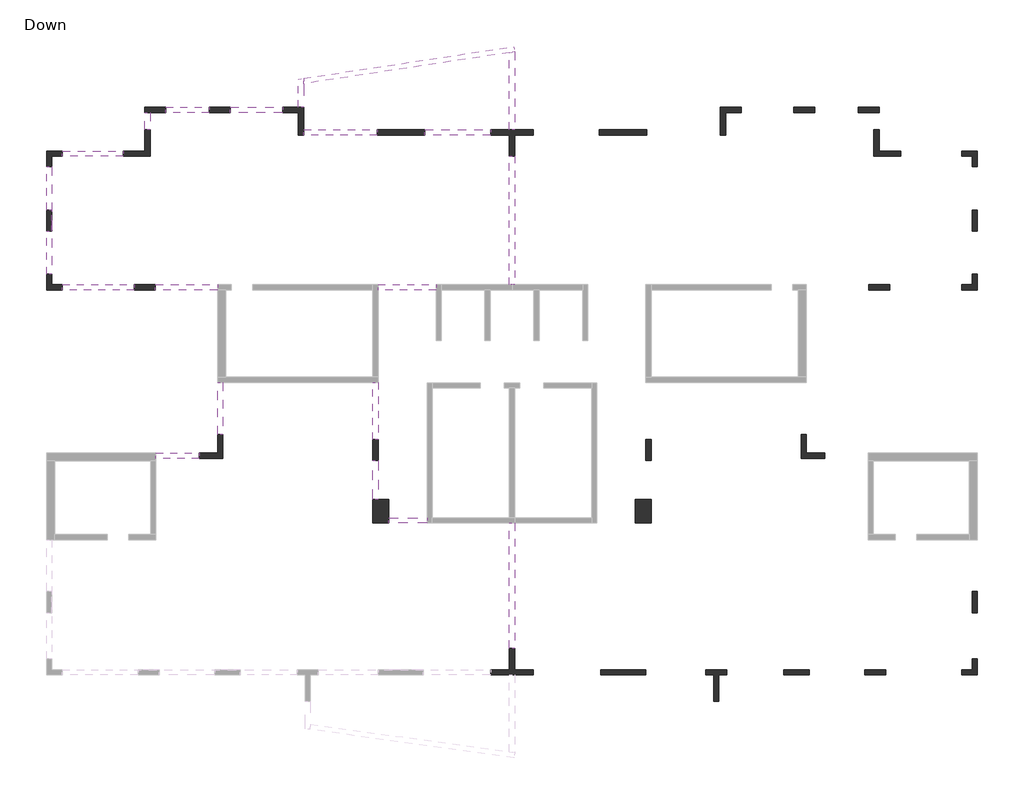
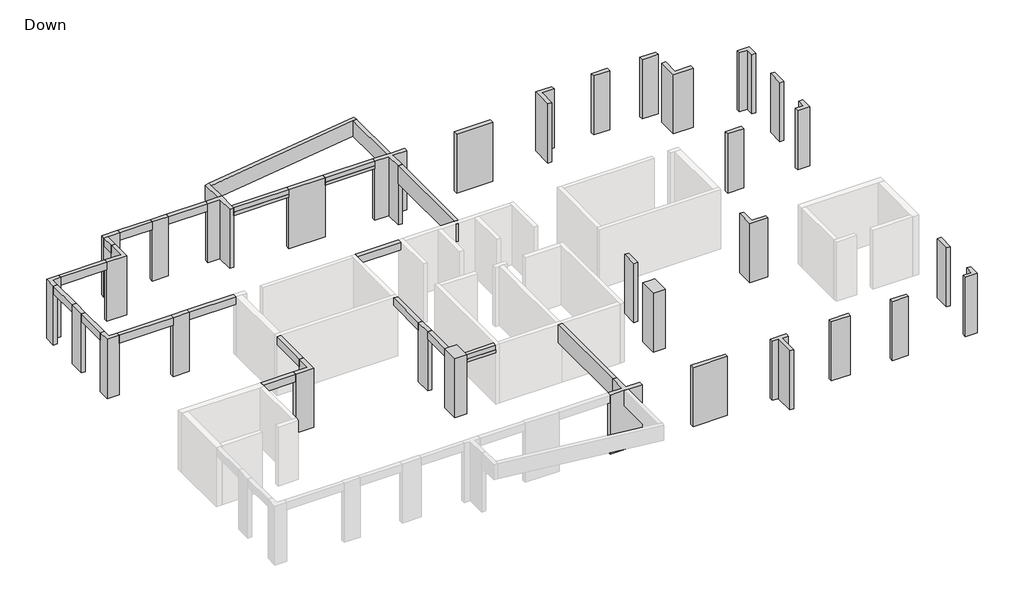
# One storey, part 2 of 2: 32 columns, 21 beams.
"""IFC4 building model written with IfcOpenShell, lengths in millimetres."""

from ifc_helpers import new_model, si_unit, frame, origin, origin_with_axes, place, context, project, spatial, polyline, outline, extrude, faceted_brep, element, save

model = new_model("IFC4")

# Units and contexts
model_context = context("Model", 3, world=origin())
ifc_project = project(units=[si_unit("LENGTHUNIT", "METRE", prefix="MILLI")], contexts=[model_context])

# Site, building, storey
site = spatial("IfcSite", under=ifc_project)
building = spatial("IfcBuilding", under=site)
storey = spatial("IfcBuildingStorey", under=building, Name="Down", Elevation=0.0)

# Beams
placement = place(None, origin())
element("IfcBeam", 1, ObjectType="Concrete Rectengular Beam : 20/40", at=placement, inside=storey, context=model_context, shape_type="Brep", body=[
    faceted_brep([(-16045.271188, -5036.9600972, 3120.0), (-16045.271188, -4836.9600972, 3120.0), (-16045.271188, -4836.9600972, 2720.0), (-16045.271188, -5036.9600972, 2720.0), (-16045.271188, -5036.9600972, 2890.0), (-14415.271188, -5036.9600972, 3120.0), (-14415.271188, -4836.9600972, 3120.0), (-14415.271188, -4836.9600972, 2720.0), (-14415.271188, -5036.9600972, 2720.0), (-14415.271188, -5036.9600972, 2890.0)], [[[0, 1, 2, 3, 4]], [[1, 0, 5, 6]], [[2, 1, 6, 7]], [[3, 2, 7, 8]], [[5, 0, 4, 3, 8, 9]], [[6, 5, 9, 8, 7]]]),
])
element("IfcBeam", 2, ObjectType="Concrete Rectengular Beam : 20/40", at=placement, inside=storey, context=model_context, shape_type="Brep", body=[
    faceted_brep([(-13715.271188, -4136.9600972, 3120.0), (-13515.271188, -4136.9600972, 3120.0), (-13515.271188, -2169.1055386, 3120.0), (-13715.271188, -2169.1055386, 3120.0), (-13515.271188, -4136.9600972, 2890.0), (-13515.271188, -4136.9600972, 2720.0), (-13515.271188, -2169.1055386, 2720.0), (-13515.271188, -2169.1055386, 2890.0), (-13715.271188, -4136.9600972, 2720.0), (-13715.271188, -2169.1055386, 2720.0)], [[[0, 1, 2, 3]], [[2, 1, 4, 5, 6, 7]], [[5, 8, 9, 6]], [[8, 0, 3, 9]], [[1, 0, 8, 5, 4]], [[3, 2, 7, 6, 9]]]),
])
element("IfcBeam", 3, ObjectType="Concrete Rectengular Beam : 20/40", at=placement, inside=storey, context=model_context, shape_type="Brep", body=[
    faceted_brep([(-5816.3023024, -7475.6540191, 2720.0), (-5816.3023024, -7475.1655965, 2720.0), (-5816.3023024, -7475.1655965, 2890.0), (-5816.3023024, -7475.6540191, 2890.0), (-5816.5012893, -7275.6540191, 3120.0), (-7266.3023024, -7275.6540191, 3120.0), (-7266.3023024, -7475.1655965, 3120.0), (-5816.5012893, -7475.1655965, 3120.0), (-7266.3023024, -7475.6540191, 2720.0), (-7266.3023024, -7475.6540191, 2890.0), (-7266.3023024, -7275.6540191, 2720.0), (-5816.5012893, -7275.6540191, 2720.0), (-5816.5012893, -7475.1655965, 2720.0), (-7266.3023024, -7275.6540191, 2890.0), (-5816.5012893, -7275.6540191, 2890.0), (-7266.3023024, -7475.1655965, 2890.0), (-5816.5012893, -7475.1655965, 2890.0)], [[[0, 1, 2, 3]], [[4, 5, 6, 7]], [[8, 0, 3, 9]], [[0, 8, 10, 11, 12, 1]], [[10, 13, 5, 4, 14, 11]], [[10, 8, 9, 15, 6, 5, 13]], [[4, 7, 16, 12, 11, 14]], [[1, 12, 16, 2]], [[16, 15, 9, 3, 2]], [[15, 16, 7, 6]]]),
])
element("IfcBeam", 4, ObjectType="Concrete Rectengular Beam : 20/40", at=placement, inside=storey, context=model_context, shape_type="Brep", body=[
    faceted_brep([(-7866.3203921, -6575.6540191, 3120.0), (-7666.3203921, -6575.6540191, 3120.0), (-7666.3203921, -5121.583831, 3120.0), (-7866.3203921, -5121.583831, 3120.0), (-7666.3203921, -6575.6540191, 2890.0), (-7666.3203921, -6575.6540191, 2720.0), (-7666.3203921, -5121.583831, 2720.0), (-7866.3203921, -6575.6540191, 2720.0), (-7866.3203921, -5121.583831, 2720.0), (-7866.3203921, -5121.583831, 2890.0), (-7866.3203921, -6575.6540191, 2890.0)], [[[0, 1, 2, 3]], [[1, 4, 5, 6, 2]], [[5, 7, 8, 6]], [[0, 3, 9, 8, 7, 10]], [[3, 2, 6, 8, 9]], [[1, 0, 10, 7, 5, 4]]]),
])
element("IfcBeam", 5, ObjectType="Concrete Rectengular Beam : 20/40", at=placement, inside=storey, context=model_context, shape_type="Brep", body=[
    faceted_brep([(-7866.3203921, -4321.583831, 3120.0), (-7666.3203921, -4321.583831, 3120.0), (-7666.3203921, -2169.1055386, 3120.0), (-7866.3203921, -2169.1055386, 3120.0), (-7666.3203921, -4321.583831, 2720.0), (-7666.3203921, -2169.1055386, 2720.0), (-7866.3203921, -4321.583831, 2720.0), (-7866.3203921, -2169.1055386, 2720.0), (-7866.3203921, -2169.1055386, 2890.0), (-7866.3203921, -4321.583831, 2890.0)], [[[0, 1, 2, 3]], [[1, 4, 5, 2]], [[4, 6, 7, 5]], [[0, 3, 8, 7, 6, 9]], [[1, 0, 9, 6, 4]], [[3, 2, 5, 7, 8]]]),
])
element("IfcBeam", 6, ObjectType="Concrete Rectengular Beam : 20/40", at=placement, inside=storey, context=model_context, shape_type="Brep", body=[
    faceted_brep([(-5479.9781345, 1313.6006842, 3120.0), (-5479.9781345, 1513.6006842, 3120.0), (-7666.3203921, 1513.6006842, 3120.0), (-7666.3203921, 1313.6006842, 3120.0), (-5479.9781345, 1313.6006842, 2720.0), (-5479.9781345, 1313.6006842, 2890.0), (-7666.3203921, 1313.6006842, 2890.0), (-7666.3203921, 1313.6006842, 2720.0), (-5479.9781345, 1513.6006842, 2720.0), (-7666.3203921, 1513.6006842, 2720.0), (-5479.9781345, 1513.6006842, 2890.0), (-7666.3203921, 1513.6006842, 2890.0)], [[[0, 1, 2, 3]], [[4, 5, 0, 3, 6, 7]], [[8, 4, 7, 9]], [[2, 1, 10, 8, 9, 11]], [[3, 2, 11, 9, 7, 6]], [[1, 0, 5, 4, 8, 10]]]),
])
element("IfcBeam", 7, ObjectType="Concrete Rectengular Beam : 20/40", at=placement, inside=storey, context=model_context, shape_type="Brep", body=[
    faceted_brep([(-16862.5034601, 1314.1252863, 3120.0), (-16862.5034601, 1514.1252863, 3120.0), (-19564.2400737, 1514.1252863, 3120.0), (-19564.2400737, 1314.1252863, 3120.0), (-16862.5034601, 1314.1252863, 2720.0), (-19564.2400737, 1314.1252863, 2720.0), (-16862.5034601, 1514.1252863, 2720.0), (-19564.2400737, 1514.1252863, 2720.0), (-16862.5034601, 1514.1252863, 2890.0)], [[[0, 1, 2, 3]], [[4, 0, 3, 5]], [[6, 4, 5, 7]], [[1, 8, 6, 7, 2]], [[1, 0, 4, 6, 8]], [[3, 2, 7, 5]]]),
])
element("IfcBeam", 8, ObjectType="Concrete Rectengular Beam : 20/40", at=placement, inside=storey, context=model_context, shape_type="Brep", body=[
    faceted_brep([(-16062.5034601, 1514.1252863, 3120.0), (-16062.5034601, 1314.1252863, 3120.0), (-13715.271188, 1314.1252863, 3120.0), (-13715.271188, 1514.1252863, 3120.0), (-16062.5034601, 1314.1252863, 2720.0), (-13715.271188, 1314.1252863, 2720.0), (-16062.5034601, 1514.1252863, 2720.0), (-13715.271188, 1514.1252863, 2720.0), (-13715.271188, 1514.1252863, 2890.0), (-16062.5034601, 1514.1252863, 2890.0)], [[[0, 1, 2, 3]], [[1, 4, 5, 2]], [[4, 6, 7, 5]], [[0, 3, 8, 7, 6, 9]], [[1, 0, 9, 6, 4]], [[3, 2, 5, 7, 8]]]),
])
element("IfcBeam", 9, ObjectType="Concrete Rectengular Beam : 20/40", at=placement, inside=storey, context=model_context, shape_type="Brep", body=[
    faceted_brep([(-19969.2400737, 3539.1252863, 3120.0), (-20164.2400737, 3539.1252863, 3120.0), (-20164.2400737, 1914.1252863, 3120.0), (-19969.2400737, 1914.1252863, 3120.0), (-19964.2400737, 3934.6498883, 2720.0), (-19964.2400737, 3934.6498883, 2890.0), (-19964.2400737, 1914.1252863, 2890.0), (-19964.2400737, 1914.1252863, 2720.0), (-19965.2892778, 3934.6498883, 2720.0), (-20164.2400737, 1914.1252863, 2720.0), (-20164.2400737, 3539.1252863, 2720.0), (-19965.2892778, 3539.1252863, 2720.0), (-19965.2892778, 3934.6498883, 2890.0), (-19965.2892778, 3539.1252863, 2890.0), (-19969.2400737, 3539.1252863, 2890.0), (-19969.2400737, 1914.1252863, 2890.0)], [[[0, 1, 2, 3]], [[4, 5, 6, 7]], [[8, 4, 7, 9, 10, 11]], [[1, 10, 9, 2]], [[4, 8, 12, 5]], [[8, 11, 13, 12]], [[11, 10, 1, 0, 14, 13]], [[5, 12, 13, 14, 15, 6]], [[14, 0, 3, 15]], [[3, 2, 9, 7, 6, 15]]]),
])
element("IfcBeam", 10, ObjectType="Concrete Rectengular Beam : 20/40", at=placement, inside=storey, context=model_context, shape_type="Brep", body=[
    faceted_brep([(-20164.2400737, 5963.5645048, 3120.0), (-20164.2400737, 4339.1252863, 3120.0), (-19969.2400737, 4339.1252863, 3120.0), (-19969.2400737, 5963.5645048, 3120.0), (-19964.2400737, 3934.6498883, 2720.0), (-19964.2400737, 5963.5645048, 2720.0), (-19964.2400737, 5963.5645048, 2890.0), (-19964.2400737, 3934.6498883, 2890.0), (-19965.2892778, 3934.6498883, 2720.0), (-19965.2892778, 4339.1252863, 2720.0), (-20164.2400737, 4339.1252863, 2720.0), (-20164.2400737, 5963.5645048, 2720.0), (-19965.2892778, 3934.6498883, 2890.0), (-19969.2400737, 5963.5645048, 2890.0), (-19965.2892778, 4339.1252863, 2890.0), (-19969.2400737, 4339.1252863, 2890.0)], [[[0, 1, 2, 3]], [[4, 5, 6, 7]], [[5, 4, 8, 9, 10, 11]], [[0, 11, 10, 1]], [[8, 4, 7, 12]], [[5, 11, 0, 3, 13, 6]], [[10, 9, 14, 15, 2, 1]], [[9, 8, 12, 14]], [[13, 15, 14, 12, 7, 6]], [[15, 13, 3, 2]]]),
])
element("IfcBeam", 11, ObjectType="Concrete Rectengular Beam : 20/40", at=placement, inside=storey, context=model_context, shape_type="Brep", body=[
    faceted_brep([(-19564.2400737, 6563.5645048, 3120.0), (-19564.2400737, 6363.5645048, 3120.0), (-17264.6018682, 6363.5645048, 3120.0), (-17264.6018682, 6563.5645048, 3120.0), (-19564.2400737, 6363.5645048, 2890.0), (-19564.2400737, 6363.5645048, 2720.0), (-17264.6018682, 6363.5645048, 2720.0), (-17264.6018682, 6363.5645048, 2890.0), (-19564.2400737, 6563.5645048, 2720.0), (-17264.6018682, 6563.5645048, 2720.0)], [[[0, 1, 2, 3]], [[2, 1, 4, 5, 6, 7]], [[5, 8, 9, 6]], [[8, 0, 3, 9]], [[1, 0, 8, 5, 4]], [[3, 2, 7, 6, 9]]]),
])
element("IfcBeam", 12, ObjectType="Concrete Rectengular Beam : 20/40", at=placement, inside=storey, context=model_context, shape_type="Brep", body=[
    faceted_brep([(-16464.6018682, 7363.5645048, 3120.0), (-16264.6018682, 7363.5645048, 3120.0), (-16264.6018682, 8012.3163138, 3120.0), (-16464.6018682, 8012.3163138, 3120.0), (-16264.6018682, 7363.5645048, 2890.0), (-16264.6018682, 7363.5645048, 2720.0), (-16264.6018682, 8012.3163138, 2720.0), (-16264.6018682, 8012.3163138, 2890.0), (-16464.6018682, 7363.5645048, 2720.0), (-16464.6018682, 8012.3163138, 2720.0)], [[[0, 1, 2, 3]], [[2, 1, 4, 5, 6, 7]], [[5, 8, 9, 6]], [[8, 0, 3, 9]], [[1, 0, 8, 5, 4]], [[3, 2, 7, 6, 9]]]),
])
element("IfcBeam", 13, ObjectType="Concrete Rectengular Beam : 20/40", at=placement, inside=storey, context=model_context, shape_type="SweptSolid", body=[
    extrude(outline(polyline([(-15664.5656888, 8012.3163138), (-15664.5656888, 8212.3163138), (-14039.0953559, 8212.3163138), (-14039.0953559, 8012.3163138), (-15664.5656888, 8012.3163138)])), frame((0.0, 0.0, 2720.0), z_axis=(0.0, 0.0, 1.0), x_axis=(1.0, 0.0, 0.0)), (0.0, 0.0, 1.0), 400.0),
])
element("IfcBeam", 14, ObjectType="Concrete Rectengular Beam : 20/40", at=placement, inside=storey, context=model_context, shape_type="SweptSolid", body=[
    extrude(outline(polyline([(-11266.4470202, 8212.3163138), (-11266.4470202, 8012.3163138), (-13239.0953559, 8012.3163138), (-13239.0953559, 8212.3163138), (-11266.4470202, 8212.3163138)])), frame((0.0, 0.0, 2720.0), z_axis=(0.0, 0.0, 1.0), x_axis=(1.0, 0.0, 0.0)), (0.0, 0.0, 1.0), 400.0),
])
element("IfcBeam", 15, ObjectType="Concrete Rectengular Beam : 20/40", at=placement, inside=storey, context=model_context, shape_type="Brep", body=[
    faceted_brep([(-7705.3941982, 7363.6006842, 3120.0), (-10466.4470202, 7363.6006842, 3120.0), (-10466.4470202, 7163.7694287, 3120.0), (-7705.3941982, 7163.7694287, 3120.0), (-10466.4470202, 7363.6006842, 2720.0), (-10466.4470202, 7363.6006842, 2890.0), (-7705.3941982, 7363.6006842, 2720.0), (-10466.4470202, 7163.6006842, 2720.0), (-7705.3941982, 7163.6006842, 2720.0), (-7705.3941982, 7163.6006842, 2890.0), (-10466.4470202, 7163.6006842, 2890.0), (-10466.4470202, 7163.7694287, 2890.0), (-7705.3941982, 7163.7694287, 2890.0)], [[[0, 1, 2, 3]], [[4, 5, 1, 0, 6]], [[7, 4, 6, 8]], [[7, 8, 9, 10]], [[1, 5, 4, 7, 10, 11, 2]], [[6, 0, 3, 12, 9, 8]], [[12, 11, 10, 9]], [[11, 12, 3, 2]]]),
])
element("IfcBeam", 16, ObjectType="Concrete Rectengular Beam : 20/40", at=placement, inside=storey, context=model_context, shape_type="SweptSolid", body=[
    extrude(outline(polyline([(7363.6006842, 2720.0), (7163.6006842, 2720.0), (7163.6006842, 2890.0), (7163.7694287, 2890.0), (7163.7694287, 3120.0), (7363.6006842, 3120.0), (7363.6006842, 2720.0)])), frame((-5905.3941982, 0.0, 0.0), z_axis=(1.0, 0.0, 0.0), x_axis=(0.0, 1.0, 0.0)), (0.0, 0.0, 1.0), 2489.0014472),
])
element("IfcBeam", 17, ObjectType="Concrete Rectengular Beam : 20/80", at=placement, inside=storey, context=model_context, shape_type="Brep", body=[
    faceted_brep([(-10466.4470202, 9303.5953834, 3120.0), (-10666.4470202, 9273.3163139, 3120.0), (-10666.4470202, 8212.3163138, 3120.0), (-10466.4470202, 8212.3163138, 3120.0), (-10466.4470202, 9101.3163136, 3120.0), (-10466.4470202, 9303.5953834, 2320.0), (-10466.4470202, 8212.3163138, 2320.0), (-10466.4470202, 9101.3163136, 2320.0), (-10666.4470202, 9273.3163139, 2320.0), (-10666.4470202, 8212.3163138, 2320.0)], [[[0, 1, 2, 3, 4]], [[5, 0, 4, 3, 6, 7]], [[8, 5, 7, 6, 9]], [[1, 8, 9, 2]], [[3, 2, 9, 6]], [[1, 0, 5, 8]]]),
])
element("IfcBeam", 18, ObjectType="Concrete Rectengular Beam : 20/80", at=placement, inside=storey, context=model_context, shape_type="Brep", body=[
    faceted_brep([(-10466.4470202, 9303.5953834, 3120.0), (-10466.4470202, 9101.3163136, 3120.0), (-2716.392751, 10274.6384721, 3120.0), (-2516.392751, 10304.9175415, 3120.0), (-2543.043603, 10480.9523568, 3120.0), (-2546.3306675, 10502.66415, 3120.0), (-2516.392751, 10304.9175415, 2320.0), (-10466.4470202, 9101.3163136, 2890.0), (-10466.4470202, 9101.3163136, 2320.0), (-2716.392751, 10274.6384721, 2320.0), (-10466.4470202, 9303.5953834, 2320.0), (-2546.3306675, 10502.66415, 2320.0), (-2543.043603, 10480.9523568, 2320.0)], [[[0, 1, 2, 3, 4, 5]], [[6, 3, 2, 1, 7, 8, 9]], [[8, 10, 11, 12, 6, 9]], [[10, 0, 5, 11]], [[1, 0, 10, 8, 7]], [[5, 4, 3, 6, 12, 11]]]),
])
element("IfcBeam", 19, ObjectType="Concrete Rectengular Beam : 20/80", at=placement, inside=storey, context=model_context, shape_type="Brep", body=[
    faceted_brep([(-2716.392751, 7363.6006842, 3120.0), (-2516.392751, 7363.6006842, 3120.0), (-2516.392751, 10274.6384721, 3120.0), (-2516.392751, 10304.9175415, 3120.0), (-2716.392751, 10274.6384721, 3120.0), (-2716.392751, 7363.6006842, 2320.0), (-2716.392751, 7363.6006842, 2890.0), (-2716.392751, 10274.6384721, 2890.0), (-2716.392751, 10274.6384721, 2320.0), (-2516.392751, 7363.6006842, 2320.0), (-2516.392751, 10304.9175415, 2320.0), (-2516.392751, 10274.6384721, 2320.0), (-2516.392751, 7363.6006842, 2890.0)], [[[0, 1, 2, 3, 4]], [[5, 6, 0, 4, 7, 8]], [[9, 5, 8, 10, 11]], [[1, 12, 9, 11, 10, 3, 2]], [[1, 0, 6, 5, 9, 12]], [[4, 3, 10, 8, 7]]]),
])
element("IfcBeam", 20, ObjectType="Concrete Rectengular Beam : 20/95", at=placement, inside=storey, context=model_context, shape_type="Brep", body=[
    faceted_brep([(-2616.3565715, 1313.6006842, 3120.0), (-2716.392751, 1313.6006842, 3120.0), (-2716.392751, 1311.2077759, 3120.0), (-2616.3565715, 1311.2077759, 3120.0), (-2716.392751, 1311.2077759, 2170.0), (-2716.392751, 1313.6006842, 2170.0), (-2616.3565715, 1313.6006842, 2170.0), (-2616.3565715, 1311.2077759, 2170.0)], [[[0, 1, 2, 3]], [[4, 2, 1, 5]], [[5, 6, 7, 4]], [[2, 4, 7, 3]], [[1, 0, 6, 5]], [[0, 3, 7, 6]]]),
    faceted_brep([(-2516.392751, 6363.6006842, 2170.0), (-2516.392751, 6363.6006842, 3120.0), (-2516.392751, 1513.6006842, 3120.0), (-2516.392751, 1513.6006842, 2890.0), (-2516.392751, 1513.6006842, 2170.0), (-2716.392751, 6363.6006842, 3120.0), (-2716.392751, 6363.6006842, 2170.0), (-2716.392751, 1513.6006842, 3120.0), (-2716.392751, 1513.6006842, 2890.0), (-2716.392751, 1513.6006842, 2170.0), (-2616.3565715, 1513.6006842, 3120.0)], [[[0, 1, 2, 3, 4]], [[5, 1, 0, 6]], [[7, 8, 9, 4, 3, 2, 10]], [[1, 5, 7, 10, 2]], [[5, 6, 9, 8, 7]], [[6, 0, 4, 9]]]),
])
element("IfcBeam", 21, ObjectType="Concrete Rectengular Beam : 20/95", at=placement, inside=storey, context=model_context, shape_type="Brep", body=[
    faceted_brep([(-2716.392751, -12204.5252202, 3120.0), (-2516.392751, -12204.5252202, 3120.0), (-2516.392751, -7475.6540191, 3120.0), (-2516.392751, -7475.1655965, 3120.0), (-2517.9484673, -7475.1655965, 3120.0), (-2716.392751, -7475.1655965, 3120.0), (-2516.392751, -12204.5252202, 2170.0), (-2516.392751, -7475.1655965, 2170.0), (-2716.392751, -12204.5252202, 2170.0), (-2716.392751, -7475.1655965, 2170.0), (-2716.392751, -7475.1655965, 2890.0)], [[[0, 1, 2, 3, 4, 5]], [[1, 6, 7, 3, 2]], [[6, 8, 9, 7]], [[8, 0, 5, 10, 9]], [[1, 0, 8, 6]], [[3, 7, 9, 10, 5, 4]]]),
])

# Columns
element("IfcColumn", 22, ObjectType="Concrete Rectengular Column : 170/20", at=placement, inside=storey, context=model_context, shape_type="Brep", body=[
    faceted_brep([(2433.5348901, -13005.5744243, 0.0), (2433.5348901, -13205.5744243, 0.0), (733.5348901, -13205.5744243, 0.0), (733.5348901, -13005.5744243, 0.0), (2433.5348901, -13005.5744243, 3120.0), (2433.5348901, -13005.5744243, 2890.0), (733.5348901, -13005.5744243, 2890.0), (733.5348901, -13005.5744243, 3120.0), (733.5348901, -13205.5744243, 2890.0), (733.5348901, -13205.5744243, 3120.0), (733.5348901, -13204.5252202, 3120.0), (733.5348901, -13009.5252202, 3120.0), (2433.5348901, -13205.5744243, 2890.0), (2433.5348901, -13205.5744243, 3120.0), (2433.5348901, -13009.5252202, 3120.0), (2433.5348901, -13204.5252202, 3120.0)], [[[0, 1, 2, 3]], [[4, 5, 0, 3, 6, 7]], [[7, 6, 3, 2, 8, 9, 10, 11]], [[9, 8, 2, 1, 12, 13]], [[13, 12, 1, 0, 5, 4, 14, 15]], [[4, 7, 11, 10, 9, 13, 15, 14]]]),
])
element("IfcColumn", 23, ObjectType="Concrete Rectengular Column : 180/20", at=placement, inside=storey, context=model_context, shape_type="Brep", body=[
    faceted_brep([(-7705.3941982, 7363.6006842, 0.0), (-5905.3941982, 7363.6006842, 0.0), (-5905.3941982, 7163.6006842, 0.0), (-7705.3941982, 7163.6006842, 0.0), (-7705.3941982, 7363.6006842, 3120.0), (-5905.3941982, 7363.6006842, 3120.0), (-5905.3941982, 7163.7694287, 3120.0), (-5905.3941982, 7163.6006842, 3120.0), (-5905.3941982, 7163.6006842, 2890.0), (-7705.3941982, 7163.6006842, 3120.0), (-7705.3941982, 7163.6006842, 2890.0), (-7705.3941982, 7163.7694287, 3120.0)], [[[0, 1, 2, 3]], [[4, 5, 1, 0]], [[5, 6, 7, 8, 2, 1]], [[7, 9, 10, 3, 2, 8]], [[9, 11, 4, 0, 3, 10]], [[4, 11, 9, 7, 6, 5]]]),
])
element("IfcColumn", 24, ObjectType="Concrete Rectengular Column : 180/20", at=placement, inside=storey, context=model_context, shape_type="Brep", body=[
    faceted_brep([(2472.6086962, 7363.6006842, 0.0), (2472.6086962, 7163.6006842, 0.0), (672.6086962, 7163.6006842, 0.0), (672.6086962, 7363.6006842, 0.0), (2472.6086962, 7363.6006842, 3120.0), (672.6086962, 7363.6006842, 3120.0), (672.6086962, 7163.6006842, 2890.0), (672.6086962, 7163.6006842, 3120.0), (672.6086962, 7168.6006842, 3120.0), (2472.6086962, 7163.6006842, 2890.0), (2472.6086962, 7163.6006842, 3120.0), (2472.6086962, 7168.6006842, 3120.0)], [[[0, 1, 2, 3]], [[4, 0, 3, 5]], [[5, 3, 2, 6, 7, 8]], [[7, 6, 2, 1, 9, 10]], [[10, 9, 1, 0, 4, 11]], [[4, 5, 8, 7, 10, 11]]]),
])
element("IfcColumn", 25, ObjectType="Concrete Rectengular Column : 80/20", at=placement, inside=storey, context=model_context, shape_type="Brep", body=[
    faceted_brep([(-16464.5656888, 8212.3163138, 0.0), (-15664.5656888, 8212.3163138, 0.0), (-15664.5656888, 8012.3163138, 0.0), (-16464.5656888, 8012.3163138, 0.0), (-16464.5656888, 8212.3163138, 3120.0), (-15664.5656888, 8212.3163138, 3120.0), (-15664.5656888, 8012.3163138, 3120.0), (-16264.6018682, 8012.3163138, 3120.0), (-16464.5656888, 8012.3163138, 3120.0)], [[[0, 1, 2, 3]], [[4, 5, 1, 0]], [[5, 6, 2, 1]], [[6, 7, 8, 3, 2]], [[8, 4, 0, 3]], [[4, 8, 7, 6, 5]]]),
])
element("IfcColumn", 26, ObjectType="Concrete Rectengular Column : 80/20", at=placement, inside=storey, context=model_context, shape_type="SweptSolid", body=[
    extrude(outline(polyline([(-14039.0953559, 8212.3163138), (-13239.0953559, 8212.3163138), (-13239.0953559, 8012.3163138), (-14039.0953559, 8012.3163138), (-14039.0953559, 8212.3163138)])), origin_with_axes(), (0.0, 0.0, 1.0), 3120.0),
])
element("IfcColumn", 27, ObjectType="Concrete Rectengular Column : 80/20", at=placement, inside=storey, context=model_context, shape_type="SweptSolid", body=[
    extrude(outline(polyline([(-16862.5034601, 1514.1252863), (-16062.5034601, 1514.1252863), (-16062.5034601, 1314.1252863), (-16862.5034601, 1314.1252863), (-16862.5034601, 1514.1252863)])), origin_with_axes(), (0.0, 0.0, 1.0), 3120.0),
])
element("IfcColumn", 28, ObjectType="Concrete Rectengular Column : 80/20", at=placement, inside=storey, context=model_context, shape_type="Brep", body=[
    faceted_brep([(-20165.2892778, 3539.1252863, 0.0), (-20165.2892778, 4339.1252863, 0.0), (-19965.2892778, 4339.1252863, 0.0), (-19965.2892778, 3539.1252863, 0.0), (-20165.2892778, 3539.1252863, 3120.0), (-20165.2892778, 4339.1252863, 3120.0), (-19969.2400737, 4339.1252863, 3120.0), (-19965.2892778, 4339.1252863, 3120.0), (-19965.2892778, 4339.1252863, 2890.0), (-19965.2892778, 3539.1252863, 3120.0), (-19965.2892778, 3539.1252863, 2890.0), (-19969.2400737, 3539.1252863, 3120.0)], [[[0, 1, 2, 3]], [[4, 5, 1, 0]], [[5, 6, 7, 8, 2, 1]], [[7, 9, 10, 3, 2, 8]], [[9, 11, 4, 0, 3, 10]], [[4, 11, 9, 7, 6, 5]]]),
])
element("IfcColumn", 29, ObjectType="Concrete Rectengular Column : 80/20", at=placement, inside=storey, context=model_context, shape_type="SweptSolid", body=[
    extrude(outline(polyline([(-7666.3203921, -4321.583831), (-7666.3203921, -5121.583831), (-7866.3203921, -5121.583831), (-7866.3203921, -4321.583831), (-7666.3203921, -4321.583831)])), origin_with_axes(), (0.0, 0.0, 1.0), 3120.0),
])
element("IfcColumn", 30, ObjectType="Concrete Rectengular Column : 80/20", at=placement, inside=storey, context=model_context, shape_type="Brep", body=[
    faceted_brep([(11231.7801868, 8212.3163138, 0.0), (11231.7801868, 8012.3163138, 0.0), (10431.7801868, 8012.3163138, 0.0), (10431.7801868, 8212.3163138, 0.0), (11231.7801868, 8212.3163138, 3120.0), (10431.7801868, 8212.3163138, 3120.0), (10431.7801868, 8012.3163138, 3120.0), (11231.7801868, 8012.3163138, 3120.0), (11031.8163662, 8012.3163138, 3120.0)], [[[0, 1, 2, 3]], [[4, 0, 3, 5]], [[5, 3, 2, 6]], [[6, 2, 1, 7, 8]], [[7, 1, 0, 4]], [[4, 5, 6, 8, 7]]]),
])
element("IfcColumn", 31, ObjectType="Concrete Rectengular Column : 80/20", at=placement, inside=storey, context=model_context, shape_type="SweptSolid", body=[
    extrude(outline(polyline([(8806.3098539, 8212.3163138), (8806.3098539, 8012.3163138), (8006.3098539, 8012.3163138), (8006.3098539, 8212.3163138), (8806.3098539, 8212.3163138)])), origin_with_axes(), (0.0, 0.0, 1.0), 3120.0),
])
element("IfcColumn", 32, ObjectType="Concrete Rectengular Column : 80/20", at=placement, inside=storey, context=model_context, shape_type="SweptSolid", body=[
    extrude(outline(polyline([(11629.7179581, 1514.1252863), (11629.7179581, 1314.1252863), (10829.7179581, 1314.1252863), (10829.7179581, 1514.1252863), (11629.7179581, 1514.1252863)])), origin_with_axes(), (0.0, 0.0, 1.0), 3120.0),
])
element("IfcColumn", 33, ObjectType="Concrete Rectengular Column : 80/20", at=placement, inside=storey, context=model_context, shape_type="Brep", body=[
    faceted_brep([(11483.6434285, -13005.8747137, 0.0), (11483.6434285, -13205.8747137, 0.0), (10683.6434285, -13205.8747137, 0.0), (10683.6434285, -13005.8747137, 0.0), (11483.6434285, -13005.8747137, 3120.0), (11483.6434285, -13005.8747137, 2890.0), (10683.6434285, -13005.8747137, 2890.0), (10683.6434285, -13005.8747137, 3120.0), (10683.6434285, -13205.8747137, 3120.0), (10683.6434285, -13009.5252202, 3120.0), (11483.6434285, -13205.8747137, 3120.0), (11483.6434285, -13009.5252202, 3120.0)], [[[0, 1, 2, 3]], [[4, 5, 0, 3, 6, 7]], [[7, 6, 3, 2, 8, 9]], [[8, 2, 1, 10]], [[10, 1, 0, 5, 4, 11]], [[4, 7, 9, 8, 10, 11]]]),
])
element("IfcColumn", 34, ObjectType="Concrete Rectengular Column : 80/20", at=placement, inside=storey, context=model_context, shape_type="Brep", body=[
    faceted_brep([(14932.5037758, 3539.1252863, 0.0), (14732.5037758, 3539.1252863, 0.0), (14732.5037758, 4339.1252863, 0.0), (14932.5037758, 4339.1252863, 0.0), (14932.5037758, 3539.1252863, 3120.0), (14932.5037758, 4339.1252863, 3120.0), (14732.5037758, 4339.1252863, 2890.0), (14732.5037758, 4339.1252863, 3120.0), (14736.4545717, 4339.1252863, 3120.0), (14732.5037758, 3539.1252863, 2890.0), (14732.5037758, 3539.1252863, 3120.0), (14736.4545717, 3539.1252863, 3120.0)], [[[0, 1, 2, 3]], [[4, 0, 3, 5]], [[5, 3, 2, 6, 7, 8]], [[7, 6, 2, 1, 9, 10]], [[10, 9, 1, 0, 4, 11]], [[4, 5, 8, 7, 10, 11]]]),
])
element("IfcColumn", 35, ObjectType="Concrete Rectengular Column : 80/20", at=placement, inside=storey, context=model_context, shape_type="SweptSolid", body=[
    extrude(outline(polyline([(14732.5037758, -10055.1764503), (14932.5037758, -10055.1764503), (14932.5037758, -10855.1764503), (14732.5037758, -10855.1764503), (14732.5037758, -10055.1764503)])), origin_with_axes(), (0.0, 0.0, 1.0), 3120.0),
])
element("IfcColumn", 36, ObjectType="Concrete Rectengular Column : 80/20", at=placement, inside=storey, context=model_context, shape_type="SweptSolid", body=[
    extrude(outline(polyline([(2433.5348901, -4321.583831), (2633.5348901, -4321.583831), (2633.5348901, -5121.583831), (2433.5348901, -5121.583831), (2433.5348901, -4321.583831)])), origin_with_axes(), (0.0, 0.0, 1.0), 3120.0),
])
element("IfcColumn", 37, ObjectType="Concrete Rectengular Column : 90/60", at=placement, inside=storey, context=model_context, shape_type="Brep", body=[
    faceted_brep([(-7266.3023024, -6575.6540191, 0.0), (-7266.3023024, -7475.6540191, 0.0), (-7866.3023024, -7475.6540191, 0.0), (-7866.3023024, -6575.6540191, 0.0), (-7266.3023024, -6575.6540191, 3120.0), (-7266.3023024, -7275.6540191, 3120.0), (-7266.3023024, -7475.1655965, 3120.0), (-7266.3023024, -7475.6540191, 3120.0), (-7266.3023024, -7475.6540191, 2890.0), (-7266.3023024, -6575.6540191, 2890.0), (-7866.3023024, -7475.6540191, 3120.0), (-7866.3023024, -7475.6540191, 2890.0), (-7866.3023024, -6575.6540191, 3120.0), (-7666.3203921, -6575.6540191, 3120.0)], [[[0, 1, 2, 3]], [[4, 5, 6, 7, 8, 1, 0, 9]], [[7, 10, 11, 2, 1, 8]], [[10, 12, 3, 2, 11]], [[12, 13, 4, 9, 0, 3]], [[4, 13, 12, 10, 7, 6, 5]]]),
])
element("IfcColumn", 38, ObjectType="Concrete Rectengular Column : 90/60", at=placement, inside=storey, context=model_context, shape_type="Brep", body=[
    faceted_brep([(2033.5168004, -6575.6540191, 0.0), (2633.5168004, -6575.6540191, 0.0), (2633.5168004, -7475.6540191, 0.0), (2033.5168004, -7475.6540191, 0.0), (2033.5168004, -6575.6540191, 3120.0), (2033.5168004, -6575.6540191, 2890.0), (2033.5168004, -7475.6540191, 3120.0), (2033.5168004, -7275.6540191, 3120.0), (2633.5168004, -7475.6540191, 2890.0), (2633.5168004, -7475.6540191, 3120.0), (2633.5168004, -6575.6540191, 3120.0), (2433.5348901, -6575.6540191, 3120.0)], [[[0, 1, 2, 3]], [[4, 5, 0, 3, 6, 7]], [[6, 3, 2, 8, 9]], [[9, 8, 2, 1, 10]], [[10, 1, 0, 5, 4, 11]], [[4, 7, 6, 9, 10, 11]]]),
])
element("IfcColumn", 39, ObjectType="Concrete Rectengular Column : 95/20", at=placement, inside=storey, context=model_context, shape_type="Brep", body=[
    faceted_brep([(8583.7700565, -13005.8747137, 0.0), (8583.7700565, -13205.8747137, 0.0), (7633.7700565, -13205.8747137, 0.0), (7633.7700565, -13005.8747137, 0.0), (8583.7700565, -13005.8747137, 3120.0), (8583.7700565, -13005.8747137, 2890.0), (7633.7700565, -13005.8747137, 2890.0), (7633.7700565, -13005.8747137, 3120.0), (7633.7700565, -13205.8747137, 3120.0), (7633.7700565, -13009.5252202, 3120.0), (8583.7700565, -13205.8747137, 3120.0), (8583.7700565, -13009.5252202, 3120.0)], [[[0, 1, 2, 3]], [[4, 5, 0, 3, 6, 7]], [[7, 6, 3, 2, 8, 9]], [[8, 2, 1, 10]], [[10, 1, 0, 5, 4, 11]], [[4, 7, 9, 8, 10, 11]]]),
])
element("IfcColumn", 40, ObjectType="L Column : 100/100/20/20", at=placement, inside=storey, context=model_context, shape_type="Brep", body=[
    faceted_brep([(-16264.6018682, 6363.5645048, 0.0), (-17264.6018682, 6363.5645048, 0.0), (-17264.6018682, 6563.5645048, 0.0), (-16464.6018682, 6563.5645048, 0.0), (-16464.6018682, 7363.5645048, 0.0), (-16264.6018682, 7363.5645048, 0.0), (-16264.6018682, 6363.5645048, 3120.0), (-17264.6018682, 6363.5645048, 3120.0), (-16264.6018682, 6363.5645048, 2890.0), (-17264.6018682, 6563.5645048, 3120.0), (-16464.6018682, 6563.5645048, 3120.0), (-16464.6018682, 7363.5645048, 3120.0), (-16264.6018682, 7363.5645048, 3120.0)], [[[0, 1, 2, 3, 4, 5]], [[6, 7, 1, 0, 8]], [[7, 9, 2, 1]], [[9, 10, 3, 2]], [[10, 11, 4, 3]], [[11, 12, 5, 4]], [[12, 6, 8, 0, 5]], [[6, 12, 11, 10, 9, 7]]]),
])
element("IfcColumn", 41, ObjectType="L Column : 105/80/20/20", at=placement, inside=storey, context=model_context, shape_type="Brep", body=[
    faceted_brep([(-10466.4470202, 8212.3163138, 0.0), (-10466.4470202, 7162.3163138, 0.0), (-10666.4470202, 7162.3163138, 0.0), (-10666.4470202, 8012.3163138, 0.0), (-11266.4470202, 8012.3163138, 0.0), (-11266.4470202, 8212.3163138, 0.0), (-10466.4470202, 8212.3163138, 3120.0), (-10466.4470202, 7363.6006842, 3120.0), (-10466.4470202, 7163.7694287, 3120.0), (-10466.4470202, 7162.3163138, 3120.0), (-10466.4470202, 7162.3163138, 2890.0), (-10666.4470202, 7162.3163138, 3120.0), (-10666.4470202, 7162.3163138, 2890.0), (-10666.4470202, 8012.3163138, 3120.0), (-10666.4470202, 8012.3163138, 2890.0), (-11266.4470202, 8012.3163138, 3120.0), (-11266.4470202, 8212.3163138, 3120.0)], [[[0, 1, 2, 3, 4, 5]], [[6, 7, 8, 9, 10, 1, 0]], [[9, 11, 12, 2, 1, 10]], [[11, 13, 14, 3, 2, 12]], [[13, 15, 4, 3, 14]], [[15, 16, 5, 4]], [[16, 6, 0, 5]], [[6, 16, 15, 13, 11, 9, 8, 7]]]),
])
element("IfcColumn", 42, ObjectType="L Column : 100/100/20/20", at=placement, inside=storey, context=model_context, shape_type="Brep", body=[
    faceted_brep([(11031.8163662, 6363.5645048, 0.0), (11031.8163662, 7363.5645048, 0.0), (11231.8163662, 7363.5645048, 0.0), (11231.8163662, 6563.5645048, 0.0), (12031.8163662, 6563.5645048, 0.0), (12031.8163662, 6363.5645048, 0.0), (11031.8163662, 6363.5645048, 3120.0), (11031.8163662, 6363.5645048, 2890.0), (12031.8163662, 6363.5645048, 3120.0), (12031.8163662, 6563.5645048, 3120.0), (11231.8163662, 6563.5645048, 3120.0), (11231.8163662, 7363.5645048, 3120.0), (11031.8163662, 7363.5645048, 3120.0)], [[[0, 1, 2, 3, 4, 5]], [[6, 7, 0, 5, 8]], [[8, 5, 4, 9]], [[9, 4, 3, 10]], [[10, 3, 2, 11]], [[11, 2, 1, 12]], [[12, 1, 0, 7, 6]], [[6, 8, 9, 10, 11, 12]]]),
])
element("IfcColumn", 43, ObjectType="L Column : 105/80/20/20", at=placement, inside=storey, context=model_context, shape_type="Brep", body=[
    faceted_brep([(5233.6615182, 8212.3163138, 0.0), (6033.6615182, 8212.3163138, 0.0), (6033.6615182, 8012.3163138, 0.0), (5433.6615182, 8012.3163138, 0.0), (5433.6615182, 7162.3163138, 0.0), (5233.6615182, 7162.3163138, 0.0), (5233.6615182, 8212.3163138, 3120.0), (5233.6615182, 7162.3163138, 2890.0), (5233.6615182, 7162.3163138, 3120.0), (5233.6615182, 7168.6006842, 3120.0), (5233.6615182, 7363.6006842, 3120.0), (5433.6615182, 7162.3163138, 2890.0), (5433.6615182, 7162.3163138, 3120.0), (5433.6615182, 8012.3163138, 2890.0), (5433.6615182, 8012.3163138, 3120.0), (6033.6615182, 8012.3163138, 3120.0), (6033.6615182, 8212.3163138, 3120.0)], [[[0, 1, 2, 3, 4, 5]], [[6, 0, 5, 7, 8, 9, 10]], [[8, 7, 5, 4, 11, 12]], [[12, 11, 4, 3, 13, 14]], [[14, 13, 3, 2, 15]], [[15, 2, 1, 16]], [[16, 1, 0, 6]], [[6, 10, 9, 8, 12, 14, 15, 16]]]),
])
element("IfcColumn", 44, ObjectType="L Column : 60/60/20/20", at=placement, inside=storey, context=model_context, shape_type="Brep", body=[
    faceted_brep([(-20164.2400737, 1314.1252863, 0.0), (-20164.2400737, 1914.1252863, 0.0), (-19964.2400737, 1914.1252863, 0.0), (-19964.2400737, 1514.1252863, 0.0), (-19564.2400737, 1514.1252863, 0.0), (-19564.2400737, 1314.1252863, 0.0), (-20164.2400737, 1314.1252863, 3120.0), (-20164.2400737, 1914.1252863, 3120.0), (-19969.2400737, 1914.1252863, 3120.0), (-19964.2400737, 1914.1252863, 3120.0), (-19964.2400737, 1914.1252863, 2890.0), (-19964.2400737, 1514.1252863, 3120.0), (-19964.2400737, 1514.1252863, 2890.0), (-19564.2400737, 1514.1252863, 3120.0), (-19564.2400737, 1314.1252863, 3120.0)], [[[0, 1, 2, 3, 4, 5]], [[6, 7, 1, 0]], [[7, 8, 9, 10, 2, 1]], [[9, 11, 12, 3, 2, 10]], [[11, 13, 4, 3, 12]], [[13, 14, 5, 4]], [[14, 6, 0, 5]], [[6, 14, 13, 11, 9, 8, 7]]]),
])
element("IfcColumn", 45, ObjectType="L Column : 60/60/20/20", at=placement, inside=storey, context=model_context, shape_type="Brep", body=[
    faceted_brep([(-20164.2400737, 6563.5645048, 0.0), (-19564.2400737, 6563.5645048, 0.0), (-19564.2400737, 6363.5645048, 0.0), (-19964.2400737, 6363.5645048, 0.0), (-19964.2400737, 5963.5645048, 0.0), (-20164.2400737, 5963.5645048, 0.0), (-20164.2400737, 6563.5645048, 3120.0), (-19564.2400737, 6563.5645048, 3120.0), (-19564.2400737, 6363.5645048, 3120.0), (-19964.2400737, 6363.5645048, 3120.0), (-19964.2400737, 6363.5645048, 2890.0), (-19964.2400737, 5963.5645048, 3120.0), (-19964.2400737, 5963.5645048, 2890.0), (-19969.2400737, 5963.5645048, 3120.0), (-20164.2400737, 5963.5645048, 3120.0)], [[[0, 1, 2, 3, 4, 5]], [[6, 7, 1, 0]], [[7, 8, 2, 1]], [[8, 9, 10, 3, 2]], [[9, 11, 12, 4, 3, 10]], [[11, 13, 14, 5, 4, 12]], [[14, 6, 0, 5]], [[6, 14, 13, 11, 9, 8, 7]]]),
])
element("IfcColumn", 46, ObjectType="L Column : 60/60/20/20", at=placement, inside=storey, context=model_context, shape_type="Brep", body=[
    faceted_brep([(14931.4545717, 1314.1252863, 0.0), (14331.4545717, 1314.1252863, 0.0), (14331.4545717, 1514.1252863, 0.0), (14731.4545717, 1514.1252863, 0.0), (14731.4545717, 1914.1252863, 0.0), (14931.4545717, 1914.1252863, 0.0), (14931.4545717, 1314.1252863, 3120.0), (14931.4545717, 1914.1252863, 3120.0), (14731.4545717, 1914.1252863, 2890.0), (14731.4545717, 1914.1252863, 3120.0), (14736.4545717, 1914.1252863, 3120.0), (14731.4545717, 1514.1252863, 2890.0), (14731.4545717, 1514.1252863, 3120.0), (14331.4545717, 1514.1252863, 3120.0), (14331.4545717, 1314.1252863, 3120.0)], [[[0, 1, 2, 3, 4, 5]], [[6, 0, 5, 7]], [[7, 5, 4, 8, 9, 10]], [[9, 8, 4, 3, 11, 12]], [[12, 11, 3, 2, 13]], [[13, 2, 1, 14]], [[14, 1, 0, 6]], [[6, 7, 10, 9, 12, 13, 14]]]),
])
element("IfcColumn", 47, ObjectType="L Column : 60/60/20/20", at=placement, inside=storey, context=model_context, shape_type="Brep", body=[
    faceted_brep([(14931.4545717, 6563.5645048, 0.0), (14931.4545717, 5963.5645048, 0.0), (14731.4545717, 5963.5645048, 0.0), (14731.4545717, 6363.5645048, 0.0), (14331.4545717, 6363.5645048, 0.0), (14331.4545717, 6563.5645048, 0.0), (14931.4545717, 6563.5645048, 3120.0), (14331.4545717, 6563.5645048, 3120.0), (14331.4545717, 6363.5645048, 3120.0), (14731.4545717, 6363.5645048, 2890.0), (14731.4545717, 6363.5645048, 3120.0), (14731.4545717, 5963.5645048, 2890.0), (14731.4545717, 5963.5645048, 3120.0), (14931.4545717, 5963.5645048, 3120.0), (14736.4545717, 5963.5645048, 3120.0)], [[[0, 1, 2, 3, 4, 5]], [[6, 0, 5, 7]], [[7, 5, 4, 8]], [[8, 4, 3, 9, 10]], [[10, 9, 3, 2, 11, 12]], [[12, 11, 2, 1, 13, 14]], [[13, 1, 0, 6]], [[6, 7, 8, 10, 12, 14, 13]]]),
])
element("IfcColumn", 48, ObjectType="L Column : 60/60/20/20", at=placement, inside=storey, context=model_context, shape_type="Brep", body=[
    faceted_brep([(14931.4545717, -13204.5252202, 0.0), (14331.4545717, -13204.5252202, 0.0), (14331.4545717, -13004.5252202, 0.0), (14731.4545717, -13004.5252202, 0.0), (14731.4545717, -12604.5252202, 0.0), (14931.4545717, -12604.5252202, 0.0), (14931.4545717, -13204.5252202, 3120.0), (14931.4545717, -12604.5252202, 3120.0), (14731.4545717, -12604.5252202, 3120.0), (14731.4545717, -13004.5252202, 2890.0), (14731.4545717, -13004.5252202, 3120.0), (14331.4545717, -13004.5252202, 2890.0), (14331.4545717, -13004.5252202, 3120.0), (14331.4545717, -13204.5252202, 3120.0), (14331.4545717, -13009.5252202, 3120.0)], [[[0, 1, 2, 3, 4, 5]], [[6, 0, 5, 7]], [[7, 5, 4, 8]], [[8, 4, 3, 9, 10]], [[10, 9, 3, 2, 11, 12]], [[12, 11, 2, 1, 13, 14]], [[13, 1, 0, 6]], [[6, 7, 8, 10, 12, 14, 13]]]),
])
element("IfcColumn", 49, ObjectType="L Column : 90/90/20/20", at=placement, inside=storey, context=model_context, shape_type="Brep", body=[
    faceted_brep([(-13515.271188, -5036.9600972, 0.0), (-14415.271188, -5036.9600972, 0.0), (-14415.271188, -4836.9600972, 0.0), (-13715.271188, -4836.9600972, 0.0), (-13715.271188, -4136.9600972, 0.0), (-13515.271188, -4136.9600972, 0.0), (-13515.271188, -5036.9600972, 3120.0), (-14415.271188, -5036.9600972, 3120.0), (-13515.271188, -5036.9600972, 2890.0), (-14415.271188, -4836.9600972, 3120.0), (-13715.271188, -4836.9600972, 3120.0), (-13715.271188, -4136.9600972, 3120.0), (-13515.271188, -4136.9600972, 3120.0)], [[[0, 1, 2, 3, 4, 5]], [[6, 7, 1, 0, 8]], [[7, 9, 2, 1]], [[9, 10, 3, 2]], [[10, 11, 4, 3]], [[11, 12, 5, 4]], [[12, 6, 8, 0, 5]], [[6, 12, 11, 10, 9, 7]]]),
])
element("IfcColumn", 50, ObjectType="L Column : 90/90/20/20", at=placement, inside=storey, context=model_context, shape_type="Brep", body=[
    faceted_brep([(8282.4856861, -5036.9600972, 0.0), (8282.4856861, -4136.9600972, 0.0), (8482.4856861, -4136.9600972, 0.0), (8482.4856861, -4836.9600972, 0.0), (9182.4856861, -4836.9600972, 0.0), (9182.4856861, -5036.9600972, 0.0), (8282.4856861, -5036.9600972, 3120.0), (8282.4856861, -5036.9600972, 2890.0), (9182.4856861, -5036.9600972, 3120.0), (9182.4856861, -4836.9600972, 3120.0), (8482.4856861, -4836.9600972, 3120.0), (8482.4856861, -4136.9600972, 3120.0), (8282.4856861, -4136.9600972, 3120.0)], [[[0, 1, 2, 3, 4, 5]], [[6, 7, 0, 5, 8]], [[8, 5, 4, 9]], [[9, 4, 3, 10]], [[10, 3, 2, 11]], [[11, 2, 1, 12]], [[12, 1, 0, 7, 6]], [[6, 8, 9, 10, 11, 12]]]),
])
element("IfcColumn", 51, ObjectType="T Column : 160/100/20/20", at=placement, inside=storey, context=model_context, shape_type="Brep", body=[
    faceted_brep([(-2516.392751, -12204.5252202, 0.0), (-2516.392751, -13004.5252202, 0.0), (-1816.392751, -13004.5252202, 0.0), (-1816.392751, -13204.5252202, 0.0), (-3416.392751, -13204.5252202, 0.0), (-3416.392751, -13004.5252202, 0.0), (-2716.392751, -13004.5252202, 0.0), (-2716.392751, -12204.5252202, 0.0), (-2516.392751, -12204.5252202, 3120.0), (-2516.392751, -13004.5252202, 3120.0), (-2516.392751, -13004.5252202, 2890.0), (-1816.392751, -13004.5252202, 3120.0), (-1816.392751, -13004.5252202, 2890.0), (-1816.392751, -13009.5252202, 3120.0), (-1816.392751, -13204.5252202, 3120.0), (-2516.392751, -13204.5252202, 3120.0), (-2716.392751, -13204.5252202, 3120.0), (-3416.392751, -13204.5252202, 3120.0), (-3416.392751, -13009.5252202, 3120.0), (-3416.392751, -13004.5252202, 3120.0), (-3416.392751, -13004.5252202, 2890.0), (-2716.392751, -13004.5252202, 3120.0), (-2716.392751, -13004.5252202, 2890.0), (-2716.392751, -12204.5252202, 3120.0)], [[[0, 1, 2, 3, 4, 5, 6, 7]], [[8, 9, 10, 1, 0]], [[9, 11, 12, 2, 1, 10]], [[11, 13, 14, 3, 2, 12]], [[14, 15, 16, 17, 4, 3]], [[17, 18, 19, 20, 5, 4]], [[19, 21, 22, 6, 5, 20]], [[21, 23, 7, 6, 22]], [[23, 8, 0, 7]], [[8, 23, 21, 19, 18, 17, 16, 15, 14, 13, 11, 9]]]),
])
element("IfcColumn", 52, ObjectType="T Column : 160/100/20/20", at=placement, inside=storey, context=model_context, shape_type="Brep", body=[
    faceted_brep([(-2716.392751, 6363.6006842, 0.0), (-2716.392751, 7163.6006842, 0.0), (-3416.392751, 7163.6006842, 0.0), (-3416.392751, 7363.6006842, 0.0), (-1816.392751, 7363.6006842, 0.0), (-1816.392751, 7163.6006842, 0.0), (-2516.392751, 7163.6006842, 0.0), (-2516.392751, 6363.6006842, 0.0), (-2716.392751, 6363.6006842, 3120.0), (-2716.392751, 7163.6006842, 3120.0), (-2716.392751, 7163.6006842, 2890.0), (-3416.392751, 7163.6006842, 3120.0), (-3416.392751, 7163.6006842, 2890.0), (-3416.392751, 7163.7694287, 3120.0), (-3416.392751, 7363.6006842, 3120.0), (-2716.392751, 7363.6006842, 3120.0), (-2516.392751, 7363.6006842, 3120.0), (-1816.392751, 7363.6006842, 3120.0), (-1816.392751, 7168.6006842, 3120.0), (-1816.392751, 7163.6006842, 3120.0), (-1816.392751, 7163.6006842, 2890.0), (-2516.392751, 7163.6006842, 3120.0), (-2516.392751, 7163.6006842, 2890.0), (-2516.392751, 6363.6006842, 3120.0)], [[[0, 1, 2, 3, 4, 5, 6, 7]], [[8, 9, 10, 1, 0]], [[9, 11, 12, 2, 1, 10]], [[11, 13, 14, 3, 2, 12]], [[14, 15, 16, 17, 4, 3]], [[17, 18, 19, 20, 5, 4]], [[19, 21, 22, 6, 5, 20]], [[21, 23, 7, 6, 22]], [[23, 8, 0, 7]], [[8, 23, 21, 19, 18, 17, 16, 15, 14, 13, 11, 9]]]),
])
element("IfcColumn", 53, ObjectType="T Column : 120/80/20/20", at=placement, inside=storey, context=model_context, shape_type="Brep", body=[
    faceted_brep([(5183.408262, -14204.5252202, 0.0), (4983.408262, -14204.5252202, 0.0), (4983.408262, -13204.5252202, 0.0), (4683.408262, -13204.5252202, 0.0), (4683.408262, -13004.5252202, 0.0), (5483.408262, -13004.5252202, 0.0), (5483.408262, -13204.5252202, 0.0), (5183.408262, -13204.5252202, 0.0), (5183.408262, -14204.5252202, 3120.0), (5183.408262, -13204.5252202, 3120.0), (5483.408262, -13204.5252202, 3120.0), (5483.408262, -13004.5252202, 2890.0), (5483.408262, -13004.5252202, 3120.0), (5483.408262, -13009.5252202, 3120.0), (4683.408262, -13004.5252202, 2890.0), (4683.408262, -13004.5252202, 3120.0), (4683.408262, -13204.5252202, 3120.0), (4683.408262, -13009.5252202, 3120.0), (4983.408262, -13204.5252202, 2890.0), (4983.408262, -13204.5252202, 3120.0), (4983.408262, -14204.5252202, 3120.0)], [[[0, 1, 2, 3, 4, 5, 6, 7]], [[8, 0, 7, 9]], [[9, 7, 6, 10]], [[10, 6, 5, 11, 12, 13]], [[12, 11, 5, 4, 14, 15]], [[15, 14, 4, 3, 16, 17]], [[16, 3, 2, 18, 19]], [[19, 18, 2, 1, 20]], [[20, 1, 0, 8]], [[8, 9, 10, 13, 12, 15, 17, 16, 19, 20]]]),
])

save(model, "model.ifc")

# Revit data of these elements
# Type "Concrete Rectengular Beam : 20/40"
#   Keynote = "09000"
#   Length [instance default] = 152.4 cm
#   b = 20 cm
#   h = 40 cm
#   Structural Material [instance default] = Concrete
#   Assembly Code = ""
# Type "Concrete Rectengular Beam : 20/80"
#   Length [instance default] = 152.4 cm
#   b = 20 cm
#   h = 80 cm
#   Structural Material [instance default] = Concrete
#   Assembly Code = ""
# Type "Concrete Rectengular Beam : 20/95"
#   Length [instance default] = 152.4 cm
#   b = 20 cm
#   h = 95 cm
#   Structural Material [instance default] = Concrete
#   Assembly Code = ""
# Type "Concrete Rectengular Column : 170/20"
#   b = 20 cm
#   h = 170 cm
#   Structural Material [instance default] = Concrete
# Type "Concrete Rectengular Column : 180/20"
#   b = 20 cm
#   h = 180 cm
#   Structural Material [instance default] = Concrete
# Type "Concrete Rectengular Column : 80/20"
#   b = 20 cm
#   h = 80 cm
#   Structural Material [instance default] = Concrete
# Type "Concrete Rectengular Column : 90/60"
#   b = 60 cm
#   h = 90 cm
#   Structural Material [instance default] = Concrete
# Type "Concrete Rectengular Column : 95/20"
#   b = 20 cm
#   h = 95 cm
#   Structural Material [instance default] = Concrete
# Type "L Column : 100/100/20/20"
#   Small Length = 20 cm
#   Small Depth = 20 cm
#   Depth = 100 cm
#   Length = 100 cm
#   Centroid Y = 90 cm
#   Centroid X = 10 cm
#   Structural Material [instance default] = Concrete, Cast-in-Place gray
# Type "L Column : 105/80/20/20"
#   Small Length = 20 cm
#   Small Depth = 20 cm
#   Depth = 80 cm
#   Length = 105 cm
#   Centroid Y = 70 cm
#   Centroid X = 10 cm
#   Structural Material [instance default] = Concrete, Cast-in-Place gray
# Type "L Column : 60/60/20/20"
#   Small Length = 20 cm
#   Small Depth = 20 cm
#   Depth = 60 cm
#   Length = 60 cm
#   Centroid Y = 50 cm
#   Centroid X = 10 cm
#   Structural Material [instance default] = Concrete, Cast-in-Place gray
# Type "L Column : 90/90/20/20"
#   Small Length = 20 cm
#   Small Depth = 20 cm
#   Depth = 90 cm
#   Length = 90 cm
#   Centroid Y = 80 cm
#   Centroid X = 10 cm
#   Structural Material [instance default] = Concrete, Cast-in-Place gray
# Type "T Column : 160/100/20/20"
#   Small Length = 20 cm
#   Small Depth = 20 cm
#   Depth = 100 cm
#   Length = 160 cm
#   Centroid Y = 90 cm
#   Centroid X from Web = 10 cm
#   Centroid X from Flange = 80 cm
#   Structural Material [instance default] = Concrete, Cast-in-Place gray
# Type "T Column : 120/80/20/20"
#   Small Length = 20 cm
#   Small Depth = 20 cm
#   Depth = 120 cm
#   Length = 80 cm
#   Centroid Y = 70 cm
#   Centroid X from Web = 10 cm
#   Centroid X from Flange = 40 cm
#   Structural Material [instance default] = Concrete, Cast-in-Place gray
# Element 1 (IfcBeam, "Concrete Rectengular Beam : 20/40")
#   Comments = ""
#   Mark = "B8"
#   SOFiSTiK_AMG_Comments = ""
#   SOFiSTiK_AMG_Scheduled = yes
#   SOFiSTiK_AMG_Adjusted = yes
#   Structural Material = Concrete
#   Phase Created = New Construction
#   Materials on its faces: "Concrete"
# Element 2 (IfcBeam, "Concrete Rectengular Beam : 20/40")
#   Comments = ""
#   Mark = "B9"
#   SOFiSTiK_AMG_Comments = ""
#   SOFiSTiK_AMG_Scheduled = yes
#   SOFiSTiK_AMG_Adjusted = yes
#   Structural Material = Concrete
#   Phase Created = New Construction
#   Materials on its faces: "Concrete"
# Element 3 (IfcBeam, "Concrete Rectengular Beam : 20/40")
#   Comments = ""
#   Mark = "B10"
#   SOFiSTiK_AMG_Comments = ""
#   SOFiSTiK_AMG_Scheduled = yes
#   SOFiSTiK_AMG_Adjusted = yes
#   Structural Material = Concrete
#   Phase Created = New Construction
#   Materials on its faces: "Concrete"
# Element 4 (IfcBeam, "Concrete Rectengular Beam : 20/40")
#   Comments = ""
#   Mark = "B11"
#   SOFiSTiK_AMG_Comments = ""
#   SOFiSTiK_AMG_Scheduled = yes
#   SOFiSTiK_AMG_Adjusted = yes
#   Structural Material = Concrete
#   Phase Created = New Construction
#   Materials on its faces: "Concrete"
# Element 5 (IfcBeam, "Concrete Rectengular Beam : 20/40")
#   Comments = ""
#   Mark = "B12"
#   SOFiSTiK_AMG_Comments = ""
#   SOFiSTiK_AMG_Scheduled = yes
#   SOFiSTiK_AMG_Adjusted = yes
#   Structural Material = Concrete
#   Phase Created = New Construction
#   Materials on its faces: "Concrete"
# Element 6 (IfcBeam, "Concrete Rectengular Beam : 20/40")
#   Comments = ""
#   Mark = "B13"
#   SOFiSTiK_AMG_Comments = ""
#   SOFiSTiK_AMG_Scheduled = yes
#   SOFiSTiK_AMG_Adjusted = yes
#   Structural Material = Concrete
#   Phase Created = New Construction
#   Materials on its faces: "Concrete"
# Element 7 (IfcBeam, "Concrete Rectengular Beam : 20/40")
#   Comments = ""
#   Mark = "B14"
#   SOFiSTiK_AMG_Comments = ""
#   SOFiSTiK_AMG_Scheduled = yes
#   SOFiSTiK_AMG_Adjusted = yes
#   Structural Material = Concrete
#   Phase Created = New Construction
#   Materials on its faces: "Concrete"
# Element 8 (IfcBeam, "Concrete Rectengular Beam : 20/40")
#   Comments = ""
#   Mark = "B15"
#   SOFiSTiK_AMG_Comments = ""
#   SOFiSTiK_AMG_Scheduled = yes
#   SOFiSTiK_AMG_Adjusted = yes
#   Structural Material = Concrete
#   Phase Created = New Construction
#   Materials on its faces: "Concrete"
# Element 9 (IfcBeam, "Concrete Rectengular Beam : 20/40")
#   Comments = ""
#   Mark = "B16"
#   SOFiSTiK_AMG_Comments = ""
#   SOFiSTiK_AMG_Scheduled = yes
#   SOFiSTiK_AMG_Adjusted = yes
#   Structural Material = Concrete
#   Phase Created = New Construction
#   Materials on its faces: "Concrete"
# Element 10 (IfcBeam, "Concrete Rectengular Beam : 20/40")
#   Comments = ""
#   Mark = "B17"
#   SOFiSTiK_AMG_Comments = ""
#   SOFiSTiK_AMG_Scheduled = yes
#   SOFiSTiK_AMG_Adjusted = yes
#   Structural Material = Concrete
#   Phase Created = New Construction
#   Materials on its faces: "Concrete"
# Element 11 (IfcBeam, "Concrete Rectengular Beam : 20/40")
#   Comments = ""
#   Mark = "B18"
#   SOFiSTiK_AMG_Comments = ""
#   SOFiSTiK_AMG_Scheduled = yes
#   SOFiSTiK_AMG_Adjusted = yes
#   Structural Material = Concrete
#   Phase Created = New Construction
#   Materials on its faces: "Concrete"
# Element 12 (IfcBeam, "Concrete Rectengular Beam : 20/40")
#   Comments = ""
#   Mark = "B19"
#   SOFiSTiK_AMG_Comments = ""
#   SOFiSTiK_AMG_Scheduled = yes
#   SOFiSTiK_AMG_Adjusted = yes
#   Structural Material = Concrete
#   Phase Created = New Construction
#   Materials on its faces: "Concrete"
# Element 13 (IfcBeam, "Concrete Rectengular Beam : 20/40")
#   Comments = ""
#   Mark = "B20"
#   SOFiSTiK_AMG_Comments = ""
#   SOFiSTiK_AMG_Scheduled = yes
#   SOFiSTiK_AMG_Adjusted = yes
#   Structural Material = Concrete
#   Phase Created = New Construction
#   Materials on its faces: "Concrete"
# Element 14 (IfcBeam, "Concrete Rectengular Beam : 20/40")
#   Comments = ""
#   Mark = "B21"
#   SOFiSTiK_AMG_Comments = ""
#   SOFiSTiK_AMG_Scheduled = yes
#   SOFiSTiK_AMG_Adjusted = yes
#   Structural Material = Concrete
#   Phase Created = New Construction
#   Materials on its faces: "Concrete"
# Element 15 (IfcBeam, "Concrete Rectengular Beam : 20/40")
#   Comments = ""
#   Mark = "B22"
#   SOFiSTiK_AMG_Comments = ""
#   SOFiSTiK_AMG_Scheduled = yes
#   SOFiSTiK_AMG_Adjusted = yes
#   Structural Material = Concrete
#   Phase Created = New Construction
#   Materials on its faces: "Concrete"
# Element 16 (IfcBeam, "Concrete Rectengular Beam : 20/40")
#   Comments = ""
#   Mark = "B23"
#   SOFiSTiK_AMG_Comments = ""
#   SOFiSTiK_AMG_Scheduled = yes
#   SOFiSTiK_AMG_Adjusted = yes
#   Structural Material = Concrete
#   Phase Created = New Construction
#   Materials on its faces: "Concrete"
# Element 17 (IfcBeam, "Concrete Rectengular Beam : 20/80")
#   Comments = ""
#   Mark = "B47"
#   SOFiSTiK_AMG_Comments = ""
#   SOFiSTiK_AMG_Scheduled = yes
#   SOFiSTiK_AMG_Adjusted = yes
#   Structural Material = Concrete
#   Phase Created = New Construction
#   Materials on its faces: "Concrete"
# Element 18 (IfcBeam, "Concrete Rectengular Beam : 20/80")
#   Comments = ""
#   Mark = "B48"
#   SOFiSTiK_AMG_Comments = ""
#   SOFiSTiK_AMG_Scheduled = yes
#   SOFiSTiK_AMG_Adjusted = yes
#   Structural Material = Concrete
#   Phase Created = New Construction
#   Materials on its faces: "Concrete"
# Element 19 (IfcBeam, "Concrete Rectengular Beam : 20/80")
#   Comments = ""
#   Mark = "B49"
#   SOFiSTiK_AMG_Comments = ""
#   SOFiSTiK_AMG_Scheduled = yes
#   SOFiSTiK_AMG_Adjusted = yes
#   Structural Material = Concrete
#   Phase Created = New Construction
#   Materials on its faces: "Concrete"
# Element 20 (IfcBeam, "Concrete Rectengular Beam : 20/95")
#   Comments = ""
#   Mark = "B57"
#   SOFiSTiK_AMG_Comments = ""
#   SOFiSTiK_AMG_Scheduled = yes
#   SOFiSTiK_AMG_Adjusted = yes
#   Structural Material = Concrete
#   Phase Created = New Construction
#   Materials on its faces: "Concrete"
# Element 21 (IfcBeam, "Concrete Rectengular Beam : 20/95")
#   Comments = ""
#   Mark = "B58"
#   SOFiSTiK_AMG_Comments = ""
#   SOFiSTiK_AMG_Scheduled = yes
#   SOFiSTiK_AMG_Adjusted = yes
#   Structural Material = Concrete
#   Phase Created = New Construction
#   Materials on its faces: "Concrete"
# Element 22 (IfcColumn, "Concrete Rectengular Column : 170/20")
#   Comments = ""
#   Mark = "C2"
#   SOFiSTiK_AMG_Comments = ""
#   SOFiSTiK_AMG_Scheduled = yes
#   SOFiSTiK_AMG_Adjusted = yes
#   Structural Material = Concrete
#   Phase Created = New Construction
#   Materials on its faces: "Concrete"
# Element 23 (IfcColumn, "Concrete Rectengular Column : 180/20")
#   Comments = ""
#   Mark = "C3"
#   SOFiSTiK_AMG_Comments = ""
#   SOFiSTiK_AMG_Scheduled = yes
#   SOFiSTiK_AMG_Adjusted = yes
#   Structural Material = Concrete
#   Phase Created = New Construction
#   Materials on its faces: "Concrete"
# Element 24 (IfcColumn, "Concrete Rectengular Column : 180/20")
#   Comments = ""
#   Mark = "C4"
#   SOFiSTiK_AMG_Comments = ""
#   SOFiSTiK_AMG_Scheduled = yes
#   SOFiSTiK_AMG_Adjusted = yes
#   Structural Material = Concrete
#   Phase Created = New Construction
#   Materials on its faces: "Concrete"
# Element 25 (IfcColumn, "Concrete Rectengular Column : 80/20")
#   Comments = ""
#   Mark = "C5"
#   SOFiSTiK_AMG_Comments = ""
#   SOFiSTiK_AMG_Scheduled = yes
#   SOFiSTiK_AMG_Adjusted = yes
#   Structural Material = Concrete
#   Phase Created = New Construction
#   Materials on its faces: "Concrete"
